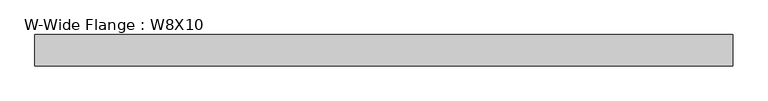
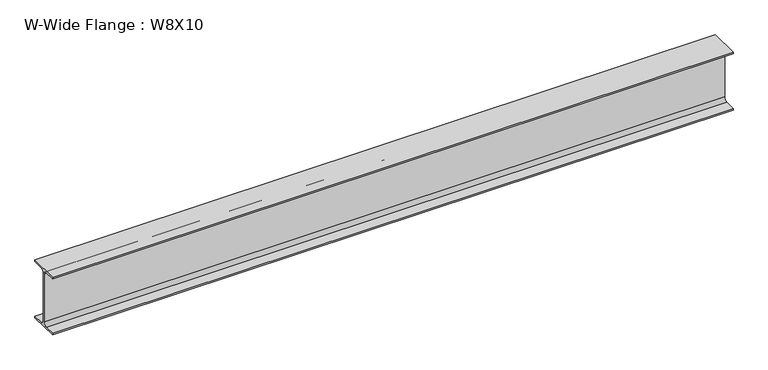
"""IFC4 building model written with IfcOpenShell, lengths in millimetres: beam geometry, W-Wide Flange : W8X10."""

from ifc_helpers import new_model, si_unit, point, frame, frame_2d, origin, place, context, project, spatial, polyline, circle_curve, trimmed, segment, composite_curve, outline, extrude, source, transform, mapped, element, save


def w_wide_flange_w8x10_c8dde3b0(model_context):
    return source(origin(), model_context, "Body", "SweptSolid", [
        extrude(outline(composite_curve([segment(polyline([(50.038, -94.996), (50.038, -100.203), (-50.038, -100.203), (-50.038, -94.996), (-14.4145, -94.996)]), True, "CONTINUOUS"), segment(trimmed(circle_curve(frame_2d((-14.4145, -82.7405)), 12.2555), [point((-14.4145, -94.996))], [point((-2.159, -82.7405))], True, "CARTESIAN"), True, "CONTINUOUS"), segment(polyline([(-2.159, -82.7405), (-2.159, 82.7405)]), True, "CONTINUOUS"), segment(trimmed(circle_curve(frame_2d((-14.4145, 82.7405)), 12.2555), [point((-2.159, 82.7405))], [point((-14.4145, 94.996))], True, "CARTESIAN"), True, "CONTINUOUS"), segment(polyline([(-14.4145, 94.996), (-50.038, 94.996), (-50.038, 100.203), (50.038, 100.203), (50.038, 94.996), (14.4145, 94.996)]), True, "CONTINUOUS"), segment(trimmed(circle_curve(frame_2d((14.4145, 82.7405)), 12.2555), [point((14.4145, 94.996))], [point((2.159, 82.7405))], True, "CARTESIAN"), True, "CONTINUOUS"), segment(polyline([(2.159, 82.7405), (2.159, -82.7405)]), True, "CONTINUOUS"), segment(trimmed(circle_curve(frame_2d((14.4145, -82.7405)), 12.2555), [point((2.159, -82.7405))], [point((14.4145, -94.996))], True, "CARTESIAN"), True, "CONTINUOUS"), segment(polyline([(14.4145, -94.996), (50.038, -94.996)]), True, "CONTINUOUS")], self_intersect=False)), frame((-1117.6, 0.0, 0.0), z_axis=(1.0, 0.0, 0.0), x_axis=(0.0, 1.0, 0.0)), (0.0, 0.0, 1.0), 2235.2),
    ])


if __name__ == "__main__":
    model = new_model("IFC4")
    model_context = context("Model", 3, world=origin())
    ifc_project = project(units=[si_unit("LENGTHUNIT", "METRE", prefix="MILLI")], contexts=[model_context])
    site = spatial("IfcSite", under=ifc_project)
    building = spatial("IfcBuilding", under=site)
    placement = place(None, origin())
    w_wide_flange_w8x10_shape = w_wide_flange_w8x10_c8dde3b0(model_context)
    element("IfcBeam", 1, ObjectType="W-Wide Flange : W8X10", at=placement, inside=building, context=model_context, shape_type="MappedRepresentation", body=[
        mapped(w_wide_flange_w8x10_shape, transform((0.0, 0.0, 0.0), x_axis=(1.0, 0.0, 0.0), y_axis=(0.0, 1.0, 0.0), z_axis=(0.0, 0.0, 1.0))),
    ])
    save(model, "model.ifc")

# Revit data of these elements
# Type "W-Wide Flange : W8X10"
#   Assembly Code = "B10"
#   W = 10
#   Length [instance default] = 5' - 0"
#   bf = 0' - 3.94"
#   d = 0' - 7.89"
#   k = 0' - 0 11/16"
#   k2 = 0' - 0.4825"
#   tf = 0' - 0.205"
#   tw = 0' - 0.17"
#   A = 0.0205556 SF
#   Structural Material [instance default] = Steel ASTM A992
# Element 1 (IfcBeam, "W-Wide Flange : W8X10")
#   Structural Material = none
# Materials
#   "Steel ASTM A992": class "Metal", colour RGB 189 187 185, transparency 0, Description = "Structural steel 50ksi", Cost = 0
